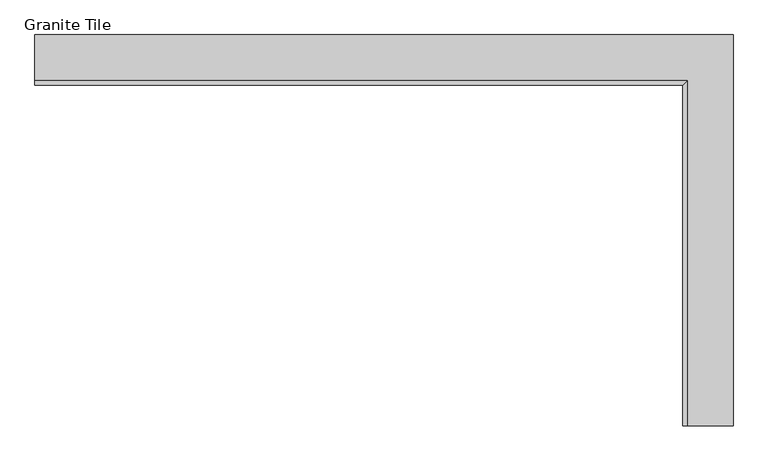
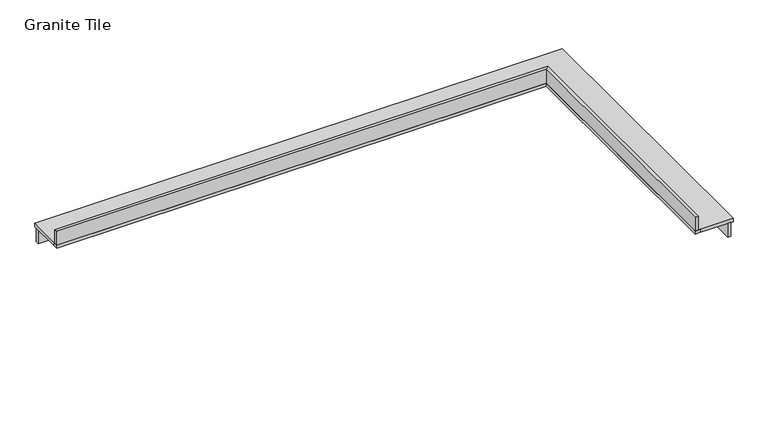
"""IFC4 building model written with IfcOpenShell, lengths in millimetres: stair flight geometry, Granite Tile."""

import ifcopenshell
import ifcopenshell.guid

model = None  # the IFC model being written
_history = None  # IfcOwnerHistory: only IFC2X3 demands one
_inside = {}  # id of a spatial element -> (the spatial element, [elements in it])
_under = {}  # id of a project, library or spatial element -> (it, [spatial elements below it])
_declared = {}  # id of a project -> (the project, [libraries it declares])
_typed = {}  # id of a type object -> (the type object, [elements of that type])
_made_of = {}  # id of a material, layer set ... -> (it, [elements and type objects made of it])


def new_model(schema):
    """Start an empty IFC model of exactly this schema.

    Asked for "IFC4X3", IfcOpenShell would pick the latest addendum, in which some entities
    have other attributes; the version numbers below select the first issue.
    IFC2X3 requires an IfcOwnerHistory on every rooted entity: one is made here for all.
    """
    global model, _history
    if schema == "IFC4X3":
        model = ifcopenshell.file(schema_version=(4, 3, 0, 0))
    else:
        model = ifcopenshell.file(schema=schema)
    _inside.clear()
    _under.clear()
    _declared.clear()
    _typed.clear()
    _made_of.clear()
    _history = None
    if model.schema == "IFC2X3":
        org = make("IfcOrganization", Name="unknown")
        user = make(
            "IfcPersonAndOrganization",
            ThePerson=make("IfcPerson", FamilyName="unknown"),
            TheOrganization=org,
        )
        app = make(
            "IfcApplication",
            ApplicationDeveloper=org,
            Version="unknown",
            ApplicationFullName="unknown",
            ApplicationIdentifier="unknown",
        )
        _history = make(
            "IfcOwnerHistory",
            OwningUser=user,
            OwningApplication=app,
            ChangeAction="ADDED",
            CreationDate=0,
        )
    return model


def make(cls, **values):
    """One entity of the class cls with the attributes given. An attribute that is None is left unset."""
    return model.create_entity(
        cls, **{name: value for name, value in values.items() if value is not None}
    )


def rooted(cls, **values):
    """An entity with a GlobalId (a new one), such as an element, a storey or a relation."""
    return make(cls, GlobalId=ifcopenshell.guid.new(), OwnerHistory=_history, **values)


def si_unit(unit_type, name, prefix=None):
    """IfcSIUnit, for example si_unit("LENGTHUNIT", "METRE", prefix="MILLI")."""
    return make("IfcSIUnit", UnitType=unit_type, Prefix=prefix, Name=name)


def assignment(units):
    """IfcUnitAssignment: the units of a project."""
    return None if units is None else make("IfcUnitAssignment", Units=units)


def point(xyz):
    """IfcCartesianPoint."""
    return None if xyz is None else make("IfcCartesianPoint", Coordinates=xyz)


def direction(xyz):
    """IfcDirection."""
    return None if xyz is None else make("IfcDirection", DirectionRatios=xyz)


def frame(location, z_axis=None, x_axis=None):
    """IfcAxis2Placement3D, a coordinate frame: its origin and axes. An axis left out is left unset."""
    return make(
        "IfcAxis2Placement3D",
        Location=point(location),
        Axis=direction(z_axis),
        RefDirection=direction(x_axis),
    )


def origin():
    """The frame at (0, 0, 0) with its axes left unset."""
    return frame((0.0, 0.0, 0.0))


def place(relative_to, where):
    """IfcLocalPlacement: puts the frame where relative to a parent placement (None: the world)."""
    return make(
        "IfcLocalPlacement", PlacementRelTo=relative_to, RelativePlacement=where
    )


def context(
    kind, dimensions, precision=None, world=None, true_north=None, identifier=None
):
    """IfcGeometricRepresentationContext, for example the 3D "Model" context."""
    return make(
        "IfcGeometricRepresentationContext",
        ContextIdentifier=identifier,
        ContextType=kind,
        CoordinateSpaceDimension=dimensions,
        Precision=precision,
        WorldCoordinateSystem=world,
        TrueNorth=true_north,
    )


def project(units=None, contexts=None):
    """IfcProject with its units and contexts."""
    return rooted(
        "IfcProject",
        Name="project",
        RepresentationContexts=contexts,
        UnitsInContext=assignment(units),
    )


def spatial(cls, under=None, at=None, **own):
    """A site, building, storey or space (cls), placed at a placement, below another one or the project."""
    s = rooted(cls, ObjectPlacement=at, **own)
    if under is not None:
        _under.setdefault(under.id(), (under, []))[1].append(s)
    return s


def faces_of(points, faces, orient=None, outer=None):
    """IfcFace entities. A face is a list of loops; a loop is a list of indices into points, from 0.

    orient and outer hold one flag for each loop. By default every Orientation is true, the
    first loop of a face is its IfcFaceOuterBound and the others are IfcFaceBound.
    """
    made = []
    for i, loops in enumerate(faces):
        bounds = []
        for j, loop in enumerate(loops):
            is_outer = j == 0 if outer is None else outer[i][j]
            bounds.append(
                make(
                    "IfcFaceOuterBound" if is_outer else "IfcFaceBound",
                    Bound=make("IfcPolyLoop", Polygon=[points[k] for k in loop]),
                    Orientation=True if orient is None else orient[i][j],
                )
            )
        made.append(make("IfcFace", Bounds=bounds))
    return made


def faceted_brep(points, faces, orient=None, outer=None, voids=None):
    """IfcFacetedBrep: a solid bounded by flat faces; with voids (closed shells), ...WithVoids."""
    shared = [point(p) for p in points]
    hull = make("IfcClosedShell", CfsFaces=faces_of(shared, faces, orient, outer))
    if voids is None:
        return make("IfcFacetedBrep", Outer=hull)
    return make(
        "IfcFacetedBrepWithVoids",
        Outer=hull,
        Voids=[
            make(cls, CfsFaces=faces_of(shared, fs, o, b)) for cls, fs, o, b in voids
        ],
    )


def shape(context_of_items, identifier, shape_type, items):
    """IfcShapeRepresentation: the items that make up one representation, for example the "Body"."""
    return make(
        "IfcShapeRepresentation",
        ContextOfItems=context_of_items,
        RepresentationIdentifier=identifier,
        RepresentationType=shape_type,
        Items=items,
    )


def source(mapping_origin, context_of_items, identifier, shape_type, items):
    """IfcRepresentationMap: a shape defined once, which mapped items show again and again."""
    return make(
        "IfcRepresentationMap",
        MappingOrigin=mapping_origin,
        MappedRepresentation=shape(context_of_items, identifier, shape_type, items),
    )


def transform(
    local_origin,
    x_axis=None,
    y_axis=None,
    z_axis=None,
    scale=None,
    scale2=None,
    scale3=None,
    uniform=True,
):
    """IfcCartesianTransformationOperator3D, or its non-uniform kind. x_axis, y_axis, z_axis: its Axis1, 2, 3."""
    if uniform:
        return make(
            "IfcCartesianTransformationOperator3D",
            Axis1=direction(x_axis),
            Axis2=direction(y_axis),
            LocalOrigin=point(local_origin),
            Scale=scale,
            Axis3=direction(z_axis),
        )
    return make(
        "IfcCartesianTransformationOperator3DnonUniform",
        Axis1=direction(x_axis),
        Axis2=direction(y_axis),
        LocalOrigin=point(local_origin),
        Scale=scale,
        Axis3=direction(z_axis),
        Scale2=scale2,
        Scale3=scale3,
    )


def mapped(mapping_source, mapping_target):
    """IfcMappedItem: shows the shape of a source again, moved by a transform."""
    return make(
        "IfcMappedItem", MappingSource=mapping_source, MappingTarget=mapping_target
    )


def made_of(thing, what):
    """Note that an element or type object is made of a material, layer set ...; save() writes the relation."""
    if what is not None:
        _made_of.setdefault(what.id(), (what, []))[1].append(thing)
    return thing


def element(
    cls,
    number,
    at=None,
    inside=None,
    cuts=None,
    type_object=None,
    material=None,
    context=None,
    identifier="Body",
    shape_type=None,
    held_by="IfcProductDefinitionShape",
    body=None,
    shapes=None,
    **own,
):
    """One element of the class cls, such as IfcWall. Its Tag is "e" and its number.

    at: its placement. inside: the storey or other place that contains it. cuts: it is an
    opening in that element (IfcRelVoidsElement). A single representation is given by context,
    identifier, shape_type and body (its items); several are given by shapes. held_by: the class
    of the entity that holds the representations. save() writes the other relations.
    """
    e = rooted(cls, Tag="e%d" % number, ObjectPlacement=at, **own)
    if body is not None:
        shapes = [shape(context, identifier, shape_type, body)]
    if shapes is not None:
        e.Representation = make(held_by, Representations=shapes)
    if inside is not None:
        _inside.setdefault(inside.id(), (inside, []))[1].append(e)
    if cuts is not None:
        rooted(
            "IfcRelVoidsElement", RelatingBuildingElement=cuts, RelatedOpeningElement=e
        )
    if type_object is not None:
        _typed.setdefault(type_object.id(), (type_object, []))[1].append(e)
    return made_of(e, material)


def aggregate(whole, parts):
    """IfcRelAggregates: a whole, such as a stair, and the parts it consists of."""
    return rooted("IfcRelAggregates", RelatingObject=whole, RelatedObjects=parts)


def save(model, path):
    """Write the relations noted so far, then the file.

    IfcRelAggregates (storeys below a building ...), IfcRelContainedInSpatialStructure (elements
    in a storey), IfcRelDefinesByType, IfcRelAssociatesMaterial and IfcRelDeclares: one each for
    every whole, place, type object, material and project.
    """
    for whole, parts in _under.values():
        aggregate(whole, parts)
    for where, things in _inside.values():
        rooted(
            "IfcRelContainedInSpatialStructure",
            RelatedElements=things,
            RelatingStructure=where,
        )
    for kind, things in _typed.values():
        rooted("IfcRelDefinesByType", RelatedObjects=things, RelatingType=kind)
    for what, things in _made_of.values():
        rooted("IfcRelAssociatesMaterial", RelatedObjects=things, RelatingMaterial=what)
    for by, libraries in _declared.values():
        rooted("IfcRelDeclares", RelatingContext=by, RelatedDefinitions=libraries)
    model.write(path)


def granite_tile_49023875(model_context):
    return source(origin(), model_context, "Body", "Brep", [
        faceted_brep([(27480.0, 300.0, 4635.0), (27450.0, 300.0, 4635.0), (27450.0, 300.0, 4500.0), (27480.0, 300.0, 4500.0), (27480.0, 3000.0, 4500.0), (27480.0, 3000.0, 4635.0), (27450.0, 2970.0, 4500.0), (27450.0, 2970.0, 4635.0), (22650.0, 3000.0, 4635.0), (22650.0, 3000.0, 4500.0), (22650.0, 2970.0, 4500.0), (22650.0, 2970.0, 4635.0)], [[[0, 1, 2, 3]], [[4, 5, 0, 3]], [[6, 4, 3, 2]], [[7, 6, 2, 1]], [[5, 7, 1, 0]], [[8, 9, 10, 11]], [[9, 8, 5, 4]], [[10, 9, 4, 6]], [[11, 10, 6, 7]], [[8, 11, 7, 5]]]),
        faceted_brep([(27150.0, 300.0, 4665.0), (27200.0, 300.0, 4665.0), (27500.0, 300.0, 4665.0), (27500.0, 3020.0, 4665.0), (22650.0, 3020.0, 4665.0), (22650.0, 2720.0, 4665.0), (22650.0, 2670.0, 4665.0), (27150.0, 2670.0, 4665.0), (27150.0, 300.0, 4635.0), (27150.0, 2670.0, 4635.0), (22650.0, 2670.0, 4635.0), (22650.0, 2720.0, 4635.0), (22650.0, 3020.0, 4635.0), (27500.0, 3020.0, 4635.0), (27500.0, 300.0, 4635.0), (27200.0, 300.0, 4635.0)], [[[0, 1, 2, 3, 4, 5, 6, 7]], [[8, 9, 10, 11, 12, 13, 14, 15]], [[1, 0, 8, 15]], [[3, 2, 14, 13]], [[5, 4, 12, 11]], [[0, 7, 9, 8]], [[4, 3, 13, 12]], [[7, 6, 10, 9]], [[2, 1, 15, 14]], [[6, 5, 11, 10]]]),
        faceted_brep([(22650.0, 2700.0, 4800.0), (22650.0, 2700.0, 4665.0), (22650.0, 2670.0, 4665.0), (22650.0, 2670.0, 4800.0), (27180.0, 2700.0, 4800.0), (27180.0, 2700.0, 4665.0), (27150.0, 2670.0, 4665.0), (27150.0, 2670.0, 4800.0), (27180.0, 300.0, 4800.0), (27150.0, 300.0, 4800.0), (27150.0, 300.0, 4665.0), (27180.0, 300.0, 4665.0)], [[[0, 1, 2, 3]], [[1, 0, 4, 5]], [[2, 1, 5, 6]], [[3, 2, 6, 7]], [[0, 3, 7, 4]], [[8, 9, 10, 11]], [[5, 4, 8, 11]], [[6, 5, 11, 10]], [[7, 6, 10, 9]], [[4, 7, 9, 8]]]),
    ])


if __name__ == "__main__":
    model = new_model("IFC4")
    model_context = context("Model", 3, world=origin())
    ifc_project = project(units=[si_unit("LENGTHUNIT", "METRE", prefix="MILLI")], contexts=[model_context])
    site = spatial("IfcSite", under=ifc_project)
    building = spatial("IfcBuilding", under=site)
    placement = place(None, origin())
    granite_tile_shape = granite_tile_49023875(model_context)
    element("IfcStairFlight", 1, ObjectType="Granite Tile", at=placement, inside=building, context=model_context, shape_type="MappedRepresentation", body=[
        mapped(granite_tile_shape, transform((0.0, 0.0, 0.0), x_axis=(1.0, 0.0, 0.0), y_axis=(0.0, 1.0, 0.0), z_axis=(0.0, 0.0, 1.0))),
    ])
    save(model, "model.ifc")

# Revit data of these elements
# Element 1 (IfcStairFlight, "Granite Tile")
#   Materials on its faces: "00_Stone_Granite"
# Materials
#   "00_Stone_Granite": class "Stone", colour RGB 99 103 98, transparency 0, Description = "Granite", Cost = 0, Image = Masonry.Stone.Granite.Square.Stacked.Polished.Black-White.jpg
